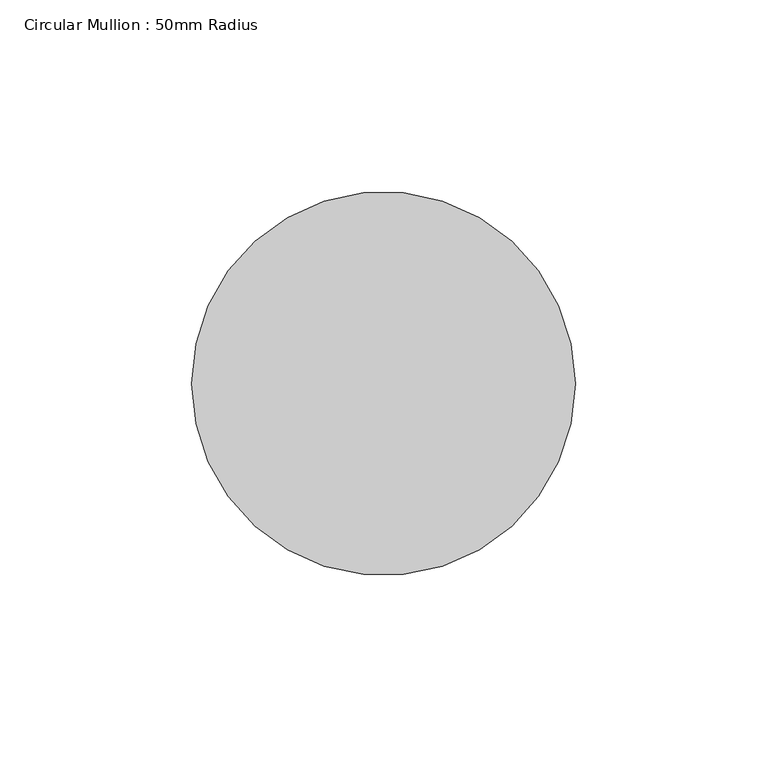
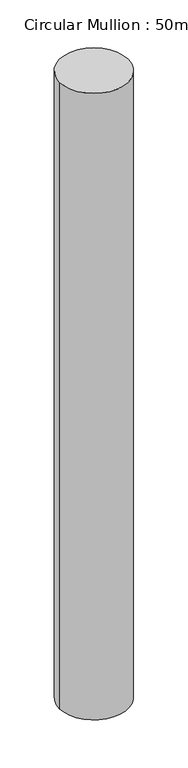
"""IFC4 building model written with IfcOpenShell, lengths in millimetres: member geometry, Circular Mullion : 50mm Radius."""

import ifcopenshell
import ifcopenshell.guid

model = None  # the IFC model being written
_history = None  # IfcOwnerHistory: only IFC2X3 demands one
_inside = {}  # id of a spatial element -> (the spatial element, [elements in it])
_under = {}  # id of a project, library or spatial element -> (it, [spatial elements below it])
_declared = {}  # id of a project -> (the project, [libraries it declares])
_typed = {}  # id of a type object -> (the type object, [elements of that type])
_made_of = {}  # id of a material, layer set ... -> (it, [elements and type objects made of it])


def new_model(schema):
    """Start an empty IFC model of exactly this schema.

    Asked for "IFC4X3", IfcOpenShell would pick the latest addendum, in which some entities
    have other attributes; the version numbers below select the first issue.
    IFC2X3 requires an IfcOwnerHistory on every rooted entity: one is made here for all.
    """
    global model, _history
    if schema == "IFC4X3":
        model = ifcopenshell.file(schema_version=(4, 3, 0, 0))
    else:
        model = ifcopenshell.file(schema=schema)
    _inside.clear()
    _under.clear()
    _declared.clear()
    _typed.clear()
    _made_of.clear()
    _history = None
    if model.schema == "IFC2X3":
        org = make("IfcOrganization", Name="unknown")
        user = make(
            "IfcPersonAndOrganization",
            ThePerson=make("IfcPerson", FamilyName="unknown"),
            TheOrganization=org,
        )
        app = make(
            "IfcApplication",
            ApplicationDeveloper=org,
            Version="unknown",
            ApplicationFullName="unknown",
            ApplicationIdentifier="unknown",
        )
        _history = make(
            "IfcOwnerHistory",
            OwningUser=user,
            OwningApplication=app,
            ChangeAction="ADDED",
            CreationDate=0,
        )
    return model


def make(cls, **values):
    """One entity of the class cls with the attributes given. An attribute that is None is left unset."""
    return model.create_entity(
        cls, **{name: value for name, value in values.items() if value is not None}
    )


def rooted(cls, **values):
    """An entity with a GlobalId (a new one), such as an element, a storey or a relation."""
    return make(cls, GlobalId=ifcopenshell.guid.new(), OwnerHistory=_history, **values)


def si_unit(unit_type, name, prefix=None):
    """IfcSIUnit, for example si_unit("LENGTHUNIT", "METRE", prefix="MILLI")."""
    return make("IfcSIUnit", UnitType=unit_type, Prefix=prefix, Name=name)


def assignment(units):
    """IfcUnitAssignment: the units of a project."""
    return None if units is None else make("IfcUnitAssignment", Units=units)


def point(xyz):
    """IfcCartesianPoint."""
    return None if xyz is None else make("IfcCartesianPoint", Coordinates=xyz)


def direction(xyz):
    """IfcDirection."""
    return None if xyz is None else make("IfcDirection", DirectionRatios=xyz)


def frame(location, z_axis=None, x_axis=None):
    """IfcAxis2Placement3D, a coordinate frame: its origin and axes. An axis left out is left unset."""
    return make(
        "IfcAxis2Placement3D",
        Location=point(location),
        Axis=direction(z_axis),
        RefDirection=direction(x_axis),
    )


def frame_2d(location, x_axis=None):
    """IfcAxis2Placement2D, a coordinate frame in the plane: its origin and x axis."""
    return make(
        "IfcAxis2Placement2D", Location=point(location), RefDirection=direction(x_axis)
    )


def origin():
    """The frame at (0, 0, 0) with its axes left unset."""
    return frame((0.0, 0.0, 0.0))


def origin_2d():
    """The frame at (0, 0) in the plane with its x axis left unset."""
    return frame_2d((0.0, 0.0))


def place(relative_to, where):
    """IfcLocalPlacement: puts the frame where relative to a parent placement (None: the world)."""
    return make(
        "IfcLocalPlacement", PlacementRelTo=relative_to, RelativePlacement=where
    )


def context(
    kind, dimensions, precision=None, world=None, true_north=None, identifier=None
):
    """IfcGeometricRepresentationContext, for example the 3D "Model" context."""
    return make(
        "IfcGeometricRepresentationContext",
        ContextIdentifier=identifier,
        ContextType=kind,
        CoordinateSpaceDimension=dimensions,
        Precision=precision,
        WorldCoordinateSystem=world,
        TrueNorth=true_north,
    )


def project(units=None, contexts=None):
    """IfcProject with its units and contexts."""
    return rooted(
        "IfcProject",
        Name="project",
        RepresentationContexts=contexts,
        UnitsInContext=assignment(units),
    )


def spatial(cls, under=None, at=None, **own):
    """A site, building, storey or space (cls), placed at a placement, below another one or the project."""
    s = rooted(cls, ObjectPlacement=at, **own)
    if under is not None:
        _under.setdefault(under.id(), (under, []))[1].append(s)
    return s


def circle_curve(where, radius):
    """IfcCircle in the frame where."""
    return make("IfcCircle", Position=where, Radius=radius)


def trimmed(basis, trim1, trim2, sense, master):
    """IfcTrimmedCurve: the piece of a basis curve between two trims."""
    return make(
        "IfcTrimmedCurve",
        BasisCurve=basis,
        Trim1=trim1,
        Trim2=trim2,
        SenseAgreement=sense,
        MasterRepresentation=master,
    )


def segment(curve, same_sense, transition):
    """IfcCompositeCurveSegment."""
    return make(
        "IfcCompositeCurveSegment",
        Transition=transition,
        SameSense=same_sense,
        ParentCurve=curve,
    )


def composite_curve(segments, self_intersect=None):
    """IfcCompositeCurve: segments joined end to end."""
    return make("IfcCompositeCurve", Segments=segments, SelfIntersect=self_intersect)


def outline(outer, holes=None, kind="AREA"):
    """IfcArbitraryClosedProfileDef: a profile drawn as a closed curve; with holes, ...WithVoids."""
    if holes is None:
        return make("IfcArbitraryClosedProfileDef", ProfileType=kind, OuterCurve=outer)
    return make(
        "IfcArbitraryProfileDefWithVoids",
        ProfileType=kind,
        OuterCurve=outer,
        InnerCurves=holes,
    )


def extrude(swept, where, along, depth):
    """IfcExtrudedAreaSolid: the profile swept, set in the frame where, extruded along a direction by depth."""
    return make(
        "IfcExtrudedAreaSolid",
        SweptArea=swept,
        Position=where,
        ExtrudedDirection=direction(along),
        Depth=depth,
    )


def shape(context_of_items, identifier, shape_type, items):
    """IfcShapeRepresentation: the items that make up one representation, for example the "Body"."""
    return make(
        "IfcShapeRepresentation",
        ContextOfItems=context_of_items,
        RepresentationIdentifier=identifier,
        RepresentationType=shape_type,
        Items=items,
    )


def source(mapping_origin, context_of_items, identifier, shape_type, items):
    """IfcRepresentationMap: a shape defined once, which mapped items show again and again."""
    return make(
        "IfcRepresentationMap",
        MappingOrigin=mapping_origin,
        MappedRepresentation=shape(context_of_items, identifier, shape_type, items),
    )


def transform(
    local_origin,
    x_axis=None,
    y_axis=None,
    z_axis=None,
    scale=None,
    scale2=None,
    scale3=None,
    uniform=True,
):
    """IfcCartesianTransformationOperator3D, or its non-uniform kind. x_axis, y_axis, z_axis: its Axis1, 2, 3."""
    if uniform:
        return make(
            "IfcCartesianTransformationOperator3D",
            Axis1=direction(x_axis),
            Axis2=direction(y_axis),
            LocalOrigin=point(local_origin),
            Scale=scale,
            Axis3=direction(z_axis),
        )
    return make(
        "IfcCartesianTransformationOperator3DnonUniform",
        Axis1=direction(x_axis),
        Axis2=direction(y_axis),
        LocalOrigin=point(local_origin),
        Scale=scale,
        Axis3=direction(z_axis),
        Scale2=scale2,
        Scale3=scale3,
    )


def mapped(mapping_source, mapping_target):
    """IfcMappedItem: shows the shape of a source again, moved by a transform."""
    return make(
        "IfcMappedItem", MappingSource=mapping_source, MappingTarget=mapping_target
    )


def made_of(thing, what):
    """Note that an element or type object is made of a material, layer set ...; save() writes the relation."""
    if what is not None:
        _made_of.setdefault(what.id(), (what, []))[1].append(thing)
    return thing


def element(
    cls,
    number,
    at=None,
    inside=None,
    cuts=None,
    type_object=None,
    material=None,
    context=None,
    identifier="Body",
    shape_type=None,
    held_by="IfcProductDefinitionShape",
    body=None,
    shapes=None,
    **own,
):
    """One element of the class cls, such as IfcWall. Its Tag is "e" and its number.

    at: its placement. inside: the storey or other place that contains it. cuts: it is an
    opening in that element (IfcRelVoidsElement). A single representation is given by context,
    identifier, shape_type and body (its items); several are given by shapes. held_by: the class
    of the entity that holds the representations. save() writes the other relations.
    """
    e = rooted(cls, Tag="e%d" % number, ObjectPlacement=at, **own)
    if body is not None:
        shapes = [shape(context, identifier, shape_type, body)]
    if shapes is not None:
        e.Representation = make(held_by, Representations=shapes)
    if inside is not None:
        _inside.setdefault(inside.id(), (inside, []))[1].append(e)
    if cuts is not None:
        rooted(
            "IfcRelVoidsElement", RelatingBuildingElement=cuts, RelatedOpeningElement=e
        )
    if type_object is not None:
        _typed.setdefault(type_object.id(), (type_object, []))[1].append(e)
    return made_of(e, material)


def aggregate(whole, parts):
    """IfcRelAggregates: a whole, such as a stair, and the parts it consists of."""
    return rooted("IfcRelAggregates", RelatingObject=whole, RelatedObjects=parts)


def save(model, path):
    """Write the relations noted so far, then the file.

    IfcRelAggregates (storeys below a building ...), IfcRelContainedInSpatialStructure (elements
    in a storey), IfcRelDefinesByType, IfcRelAssociatesMaterial and IfcRelDeclares: one each for
    every whole, place, type object, material and project.
    """
    for whole, parts in _under.values():
        aggregate(whole, parts)
    for where, things in _inside.values():
        rooted(
            "IfcRelContainedInSpatialStructure",
            RelatedElements=things,
            RelatingStructure=where,
        )
    for kind, things in _typed.values():
        rooted("IfcRelDefinesByType", RelatedObjects=things, RelatingType=kind)
    for what, things in _made_of.values():
        rooted("IfcRelAssociatesMaterial", RelatedObjects=things, RelatingMaterial=what)
    for by, libraries in _declared.values():
        rooted("IfcRelDeclares", RelatingContext=by, RelatedDefinitions=libraries)
    model.write(path)


def circular_mullion_50mm_radius_4aa5fdd3(model_context):
    return source(origin(), model_context, "Body", "SweptSolid", [
        extrude(outline(composite_curve([segment(trimmed(circle_curve(origin_2d(), 50.0), [point((50.0, 0.0))], [point((-50.0, 0.0))], False, "CARTESIAN"), True, "CONTINUOUS"), segment(trimmed(circle_curve(origin_2d(), 50.0), [point((-50.0, 0.0))], [point((50.0, 0.0))], False, "CARTESIAN"), True, "CONTINUOUS")], self_intersect=False)), frame((0.0, 0.0, -964.4626834), z_axis=(0.0, 0.0, 1.0), x_axis=(1.0, 0.0, 0.0)), (0.0, 0.0, 1.0), 964.4626834),
    ])


if __name__ == "__main__":
    model = new_model("IFC4")
    model_context = context("Model", 3, world=origin())
    ifc_project = project(units=[si_unit("LENGTHUNIT", "METRE", prefix="MILLI")], contexts=[model_context])
    site = spatial("IfcSite", under=ifc_project)
    building = spatial("IfcBuilding", under=site)
    placement = place(None, origin())
    circular_mullion_50mm_radius_shape = circular_mullion_50mm_radius_4aa5fdd3(model_context)
    element("IfcMember", 1, ObjectType="Circular Mullion : 50mm Radius", at=placement, inside=building, context=model_context, shape_type="MappedRepresentation", body=[
        mapped(circular_mullion_50mm_radius_shape, transform((0.0, 0.0, 0.0), x_axis=(1.0, 0.0, 0.0), y_axis=(0.0, 1.0, 0.0), z_axis=(0.0, 0.0, 1.0))),
    ])
    save(model, "model.ifc")

# Revit data of these elements
# Type "Circular Mullion : 50mm Radius"
#   built-in parameter 1007350 = 0.164042 (stored number, unit not read)
# Element 1 (IfcMember, "Circular Mullion : 50mm Radius")
#   Materials on its faces: "Aluminium"
# Materials
#   "Aluminium": class "Metal", colour RGB 247 247 247, transparency 0, Description = "Aluminium 6061", Cost = 0
